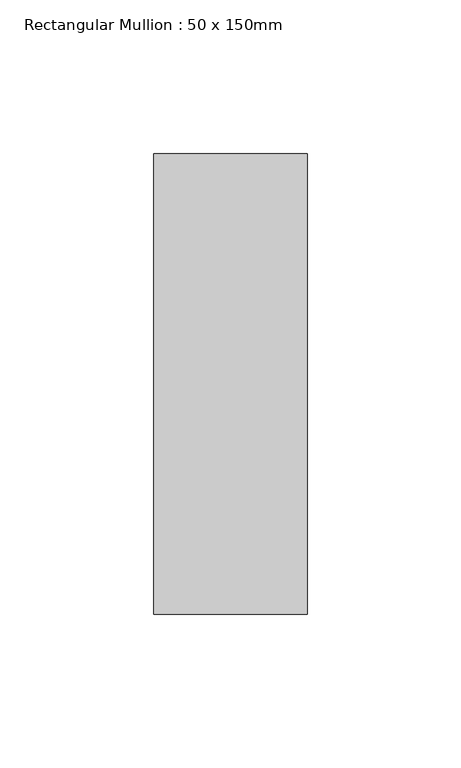
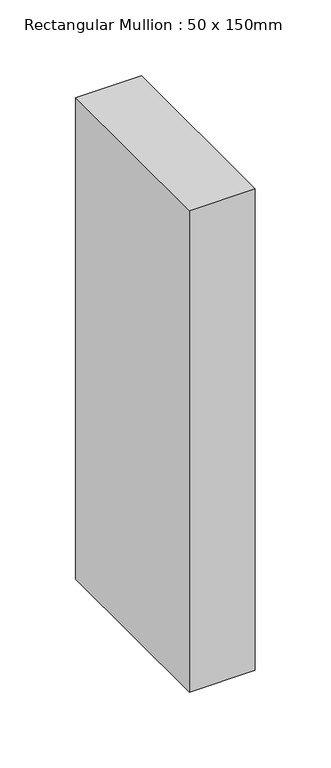
"""IFC4 building model written with IfcOpenShell, lengths in millimetres: member geometry, Rectangular Mullion : 50 x 150mm."""

from ifc_helpers import new_model, si_unit, frame, origin, place, context, project, spatial, polyline, outline, extrude, source, transform, mapped, element, save


def rectangular_mullion_50_x_150mm_e3c12dcf(model_context):
    return source(origin(), model_context, "Body", "SweptSolid", [
        extrude(outline(polyline([(0.0, 75.0), (0.0, -75.0), (-50.0, -75.0), (-50.0, 75.0), (0.0, 75.0)])), frame((0.0, 0.0, -387.5), z_axis=(0.0, 0.0, 1.0), x_axis=(1.0, 0.0, 0.0)), (0.0, 0.0, 1.0), 387.5),
    ])


if __name__ == "__main__":
    model = new_model("IFC4")
    model_context = context("Model", 3, world=origin())
    ifc_project = project(units=[si_unit("LENGTHUNIT", "METRE", prefix="MILLI")], contexts=[model_context])
    site = spatial("IfcSite", under=ifc_project)
    building = spatial("IfcBuilding", under=site)
    placement = place(None, origin())
    rectangular_mullion_50_x_150mm_shape = rectangular_mullion_50_x_150mm_e3c12dcf(model_context)
    element("IfcMember", 1, ObjectType="Rectangular Mullion : 50 x 150mm", at=placement, inside=building, context=model_context, shape_type="MappedRepresentation", body=[
        mapped(rectangular_mullion_50_x_150mm_shape, transform((0.0, 0.0, 0.0), x_axis=(1.0, 0.0, 0.0), y_axis=(0.0, 1.0, 0.0), z_axis=(0.0, 0.0, 1.0))),
    ])
    save(model, "model.ifc")

# Revit data of these elements
# Type "Rectangular Mullion : 50 x 150mm"
#   built-in parameter 1007304 = 0.492126 (stored number, unit not read)
#   built-in parameter 1007301 = 0.082021 (stored number, unit not read)
#   built-in parameter 1007300 = 0.082021 (stored number, unit not read)
# Element 1 (IfcMember, "Rectangular Mullion : 50 x 150mm")
#   Materials on its faces: "Aluminium"
# Materials
#   "Aluminium": class "Metal", colour RGB 247 247 247, transparency 0, Description = "Aluminium 6061", Cost = 0
